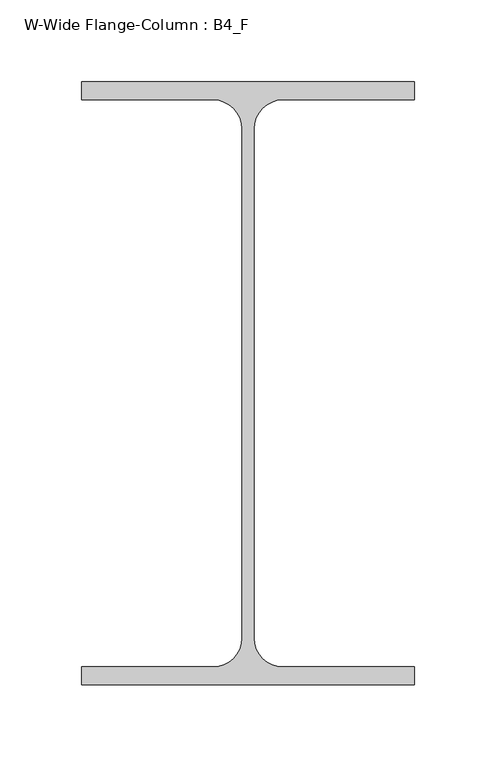
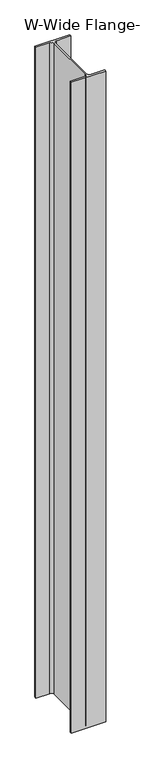
"""IFC4 building model written with IfcOpenShell, lengths in millimetres: column geometry, W-Wide Flange-Column : B4_F."""

from ifc_helpers import new_model, si_unit, point, frame, frame_2d, origin, place, context, project, spatial, polyline, circle_curve, trimmed, segment, composite_curve, outline, extrude, source, transform, mapped, element, save


def w_wide_flange_column_b4_f_8a8a01a4(model_context):
    return source(origin(), model_context, "Body", "SweptSolid", [
        extrude(outline(composite_curve([segment(polyline([(101.6, 184.15), (101.6, 173.1367188), (21.2328125, 173.1367188)]), True, "CONTINUOUS"), segment(trimmed(circle_curve(frame_2d((21.2328125, 155.575)), 17.5617188), [point((21.2328125, 173.1367188))], [point((3.6710937, 155.575))], True, "CARTESIAN"), True, "CONTINUOUS"), segment(polyline([(3.6710937, 155.575), (3.6710937, -155.575)]), True, "CONTINUOUS"), segment(trimmed(circle_curve(frame_2d((21.2328125, -155.575)), 17.5617188), [point((3.6710937, -155.575))], [point((21.2328125, -173.1367187))], True, "CARTESIAN"), True, "CONTINUOUS"), segment(polyline([(21.2328125, -173.1367187), (101.6, -173.1367187), (101.6, -184.15), (-101.6, -184.15), (-101.6, -173.1367187), (-21.2328125, -173.1367187)]), True, "CONTINUOUS"), segment(trimmed(circle_curve(frame_2d((-21.2328125, -155.575)), 17.5617188), [point((-21.2328125, -173.1367187))], [point((-3.6710938, -155.575))], True, "CARTESIAN"), True, "CONTINUOUS"), segment(polyline([(-3.6710938, -155.575), (-3.6710938, 155.575)]), True, "CONTINUOUS"), segment(trimmed(circle_curve(frame_2d((-21.2328125, 155.575)), 17.5617188), [point((-3.6710938, 155.575))], [point((-21.2328125, 173.1367188))], True, "CARTESIAN"), True, "CONTINUOUS"), segment(polyline([(-21.2328125, 173.1367188), (-101.6, 173.1367188), (-101.6, 184.15), (101.6, 184.15)]), True, "CONTINUOUS")], self_intersect=False)), frame((0.0, 0.0, -304.8), z_axis=(0.0, 0.0, 1.0), x_axis=(1.0, 0.0, 0.0)), (0.0, 0.0, 1.0), 4025.9),
    ])


if __name__ == "__main__":
    model = new_model("IFC4")
    model_context = context("Model", 3, world=origin())
    ifc_project = project(units=[si_unit("LENGTHUNIT", "METRE", prefix="MILLI")], contexts=[model_context])
    site = spatial("IfcSite", under=ifc_project)
    building = spatial("IfcBuilding", under=site)
    placement = place(None, origin())
    w_wide_flange_column_b4_f_shape = w_wide_flange_column_b4_f_8a8a01a4(model_context)
    element("IfcColumn", 1, ObjectType="W-Wide Flange-Column : B4_F", at=placement, inside=building, context=model_context, shape_type="MappedRepresentation", body=[
        mapped(w_wide_flange_column_b4_f_shape, transform((0.0, 0.0, 0.0), x_axis=(1.0, 0.0, 0.0), y_axis=(0.0, 1.0, 0.0), z_axis=(0.0, 0.0, 1.0))),
    ])
    save(model, "model.ifc")

# Revit data of these elements
# Type "W-Wide Flange-Column : B4_F"
#   Assembly Code = "B10"
#   W = 33
#   bf = 0' - 8"
#   d = 1' - 2 1/2"
#   k = 0' - 1 1/8"
#   kr = 0' - 0 177/256"
#   tf = 0' - 0 111/256"
#   tw = 0' - 0 37/128"
#   A = 0.07 SF
#   Structural Material [instance default] = Steel ASTM A992
# Element 1 (IfcColumn, "W-Wide Flange-Column : B4_F")
#   Structural Material = STRUCTURAL STEEL - SEE STRUCT. DWGS
#   Materials on its faces: "STRUCTURAL STEEL - SEE STRUCT. DWGS"
# Materials
#   "Steel ASTM A992": class "Metal", colour RGB 199 199 199, transparency 0, Description = "Structural steel 50ksi", Cost = 0
#   "STRUCTURAL STEEL - SEE STRUCT. DWGS": class "Metal", colour RGB 137 146 153, transparency 0, Description = "Steel, mill finish", Cost = 0
